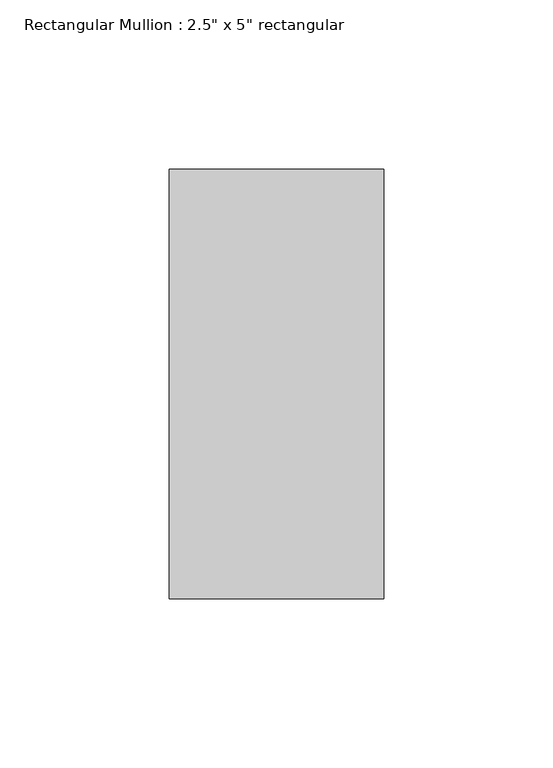
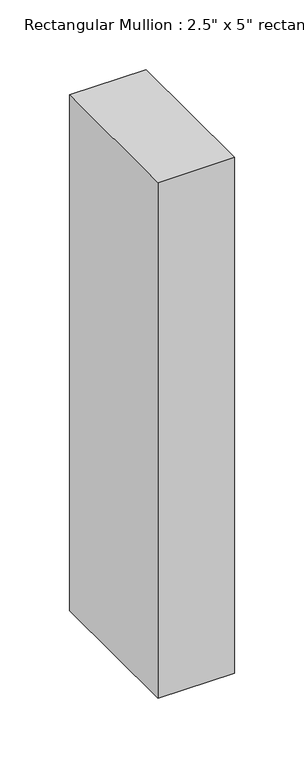
"""IFC4 building model written with IfcOpenShell, lengths in millimetres: member geometry."""

from ifc_helpers import new_model, si_unit, frame, origin, place, context, project, spatial, polyline, outline, extrude, source, transform, mapped, element, save


def member_337a90be(model_context):
    return source(origin(), model_context, "Body", "SweptSolid", [
        extrude(outline(polyline([(0.0, 63.5), (0.0, -63.5), (-63.5, -63.5), (-63.5, 63.5), (0.0, 63.5)])), frame((0.0, 0.0, -451.964047), z_axis=(0.0, 0.0, 1.0), x_axis=(1.0, 0.0, 0.0)), (0.0, 0.0, 1.0), 451.964047),
    ])


if __name__ == "__main__":
    model = new_model("IFC4")
    model_context = context("Model", 3, world=origin())
    ifc_project = project(units=[si_unit("LENGTHUNIT", "METRE", prefix="MILLI")], contexts=[model_context])
    site = spatial("IfcSite", under=ifc_project)
    building = spatial("IfcBuilding", under=site)
    placement = place(None, origin())
    member_shape = member_337a90be(model_context)
    element("IfcMember", 1, ObjectType="Rectangular Mullion : 2.5\" x 5\" rectangular", at=placement, inside=building, context=model_context, shape_type="MappedRepresentation", body=[
        mapped(member_shape, transform((0.0, 0.0, 0.0), x_axis=(1.0, 0.0, 0.0), y_axis=(0.0, 1.0, 0.0), z_axis=(0.0, 0.0, 1.0))),
    ])
    save(model, "model.ifc")

# Revit data of these elements
# Type "Rectangular Mullion : 2.5\" x 5\" rectangular"
#   built-in parameter 1007304 = 0.416667 (stored number, unit not read)
#   built-in parameter 1007301 = 0.104167 (stored number, unit not read)
#   built-in parameter 1007300 = 0.104167 (stored number, unit not read)
# Element 1 (IfcMember, "Rectangular Mullion : 2.5\" x 5\" rectangular")
#   Materials on its faces: "Metal - Aluminum 2"
# Materials
#   "Metal - Aluminum 2": class "Metal", colour RGB 189 187 185, transparency 0
